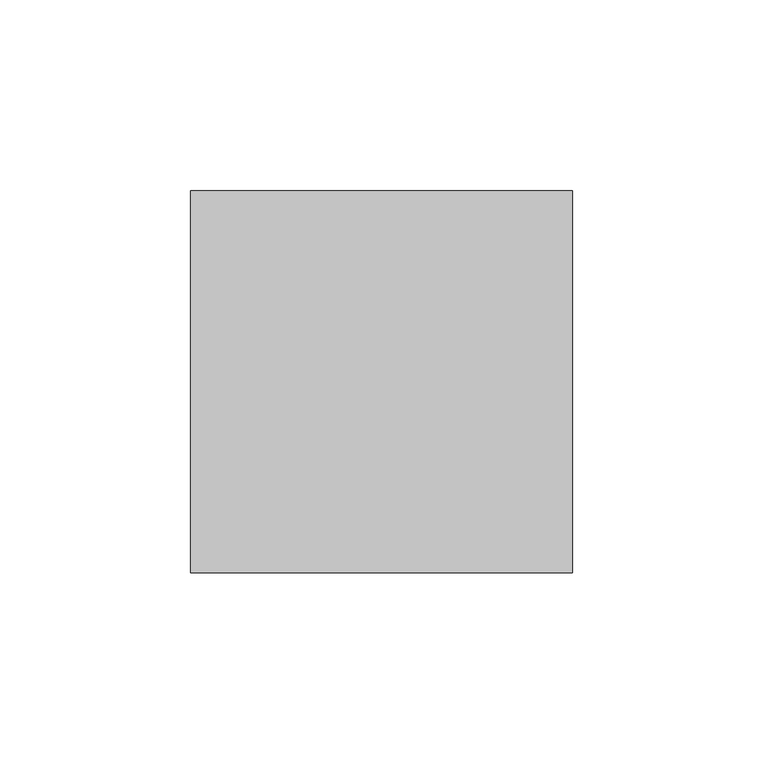
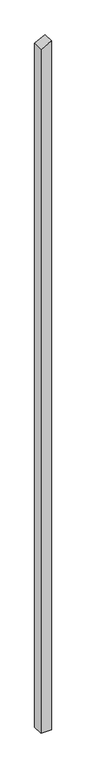
"""IFC4 building model written with IfcOpenShell, lengths in millimetres: column geometry, Holzstütze 160006 : Holzstütze 160006."""

from ifc_helpers import new_model, si_unit, frame, origin, place, context, project, spatial, polyline, outline, extrude, source, transform, mapped, element, save


def column_65cb31a2(model_context):
    return source(origin(), model_context, "Body", "SweptSolid", [
        extrude(outline(polyline([(-500.0, 157297.7593015), (-500.0, 157397.7593015), (6396.6643707, 157397.7593015), (6345.7118258, 157297.7593015), (-500.0, 157297.7593015)])), frame((0.0, 29551.5369795, 0.0), z_axis=(0.0, 1.0, 0.0), x_axis=(0.0, 0.0, 1.0)), (0.0, 0.0, 1.0), 100.0),
    ])


if __name__ == "__main__":
    model = new_model("IFC4")
    model_context = context("Model", 3, world=origin())
    ifc_project = project(units=[si_unit("LENGTHUNIT", "METRE", prefix="MILLI")], contexts=[model_context])
    site = spatial("IfcSite", under=ifc_project)
    building = spatial("IfcBuilding", under=site)
    placement = place(None, origin())
    column_shape = column_65cb31a2(model_context)
    element("IfcColumn", 1, ObjectType="Holzstütze 160006 : Holzstütze 160006", at=placement, inside=building, context=model_context, shape_type="MappedRepresentation", body=[
        mapped(column_shape, transform((0.0, 0.0, 0.0), x_axis=(1.0, 0.0, 0.0), y_axis=(0.0, 1.0, 0.0), z_axis=(0.0, 0.0, 1.0))),
    ])
    save(model, "model.ifc")

# Revit data of these elements
# Type "Holzstütze 160006 : Holzstütze 160006"
#   Abrechnungsart = "m"
#   Allright_Bauteil_ID = "0152St 0000143504"
#   Bezeichnung = "Holzstütze"
#   Codetext = "ST-HOLZ\\"
#   Gewerk = "Zimmer- und Holzbauarbeiten"
#   Material = "Holz"
#   Objektname = "Stütze"
#   NameOverride = "Holzstütze"
#   Reference = "Holzstütze"
#   Status = "NEW"
#   ThermalTransmittance = 0.0000 BTU/(h·ft²·°F)
#   Roll = 0.00°
#   Slope = 0.00°
#   2D Interaktion = yes
#   IsExternal = yes
#   LoadBearing = yes
# Element 1 (IfcColumn, "Holzstütze 160006 : Holzstütze 160006")
#   Materials on its faces: "holzschalung"
# Materials
#   "holzschalung": class "Unassigned", colour RGB 128 128 128, transparency 0
